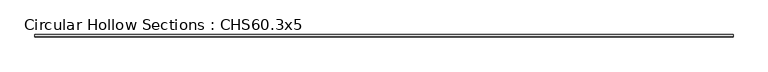
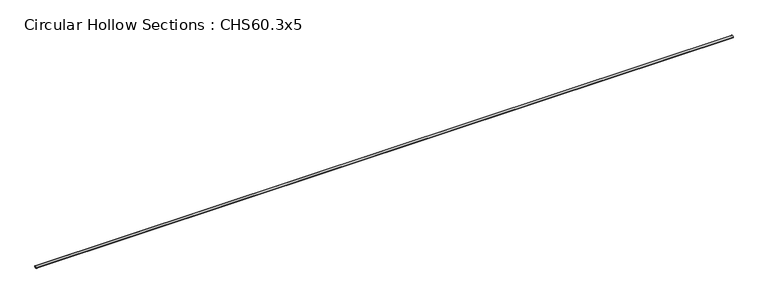
"""IFC4 building model written with IfcOpenShell, lengths in millimetres: beam geometry, Circular Hollow Sections : CHS60.3x5."""

from ifc_helpers import new_model, si_unit, point, frame, origin, origin_2d, place, context, project, spatial, circle_curve, trimmed, segment, composite_curve, outline, extrude, source, transform, mapped, element, save


def circular_hollow_sections_chs60_3x5_ee2473de(model_context):
    return source(origin(), model_context, "Body", "SweptSolid", [
        extrude(outline(composite_curve([segment(trimmed(circle_curve(origin_2d(), 30.15), [point((-30.15, 0.0))], [point((30.15, 0.0))], False, "CARTESIAN"), True, "CONTINUOUS"), segment(trimmed(circle_curve(origin_2d(), 30.15), [point((30.15, 0.0))], [point((-30.15, 0.0))], False, "CARTESIAN"), True, "CONTINUOUS")], self_intersect=False), holes=[composite_curve([segment(trimmed(circle_curve(origin_2d(), 25.15), [point((25.15, 0.0))], [point((-25.15, 0.0))], True, "CARTESIAN"), True, "CONTINUOUS"), segment(trimmed(circle_curve(origin_2d(), 25.15), [point((-25.15, 0.0))], [point((25.15, 0.0))], True, "CARTESIAN"), True, "CONTINUOUS")], self_intersect=False)]), frame((-9000.0, 0.0, 0.0), z_axis=(1.0, 0.0, 0.0), x_axis=(0.0, 1.0, 0.0)), (0.0, 0.0, 1.0), 18000.0),
    ])


if __name__ == "__main__":
    model = new_model("IFC4")
    model_context = context("Model", 3, world=origin())
    ifc_project = project(units=[si_unit("LENGTHUNIT", "METRE", prefix="MILLI")], contexts=[model_context])
    site = spatial("IfcSite", under=ifc_project)
    building = spatial("IfcBuilding", under=site)
    placement = place(None, origin())
    circular_hollow_sections_chs60_3x5_shape = circular_hollow_sections_chs60_3x5_ee2473de(model_context)
    element("IfcBeam", 1, ObjectType="Circular Hollow Sections : CHS60.3x5", at=placement, inside=building, context=model_context, shape_type="MappedRepresentation", body=[
        mapped(circular_hollow_sections_chs60_3x5_shape, transform((0.0, 0.0, 0.0), x_axis=(1.0, 0.0, 0.0), y_axis=(0.0, 1.0, 0.0), z_axis=(0.0, 0.0, 1.0))),
    ])
    save(model, "model.ifc")

# Revit data of these elements
# Type "Circular Hollow Sections : CHS60.3x5"
#   Description = "Hollow Core Steel Roof Truss Member"
#   Type Comments = "Steel 50-355"
#   Assembly Code = "F10"
#   t = 5 mm
#   W = 0.00682
#   Start Extension Calculation [instance default] = 3000 mm
#   Start Extension [instance default] = -12.7 mm
#   Length [instance default] = 1500 mm
#   OD = 60.3 mm
#   End Extension Calculation [instance default] = 3000 mm
#   End Extension [instance default] = -12.7 mm
#   A = 0.000869 m²
#   Structural Material [instance default] = Metal - Steel 50-355
# Element 1 (IfcBeam, "Circular Hollow Sections : CHS60.3x5")
#   Materials on its faces: "Metal - Steel 50-355"
# Materials
#   "Metal - Steel 50-355": class "Metal", colour RGB 247 247 247, transparency 0
